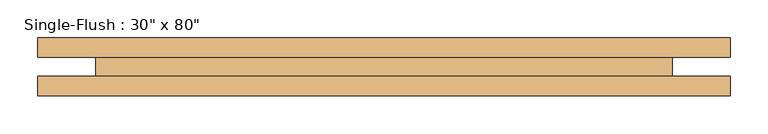
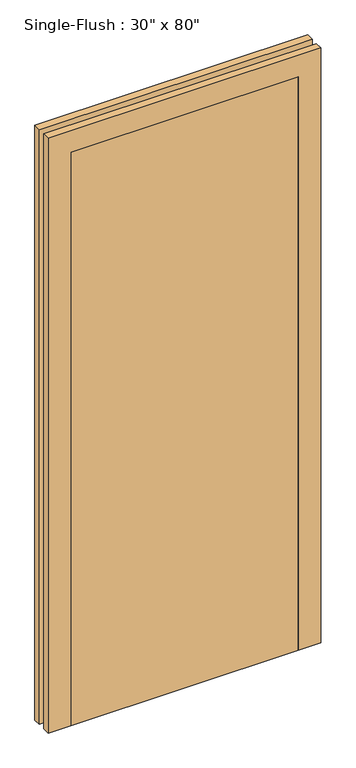
"""IFC4 building model written with IfcOpenShell, lengths in millimetres: door geometry."""

from ifc_helpers import new_model, si_unit, frame, origin, origin_with_axes, place, context, project, spatial, polyline, outline, extrude, source, transform, mapped, element, save


def door_b03708da(model_context):
    return source(origin(), model_context, "Body", "SweptSolid", [
        extrude(outline(polyline([(2108.2, -457.2), (0.0, -457.2), (0.0, -381.0), (2032.0, -381.0), (2032.0, 381.0), (0.0, 381.0), (0.0, 457.2), (2108.2, 457.2), (2108.2, -457.2)])), frame((0.0, 12.7, 0.0), z_axis=(0.0, 1.0, 0.0), x_axis=(0.0, 0.0, 1.0)), (0.0, 0.0, 1.0), 25.4),
        extrude(outline(polyline([(2108.2, 457.2), (2108.2, -457.2), (0.0, -457.2), (0.0, -381.0), (2032.0, -381.0), (2032.0, 381.0), (0.0, 381.0), (0.0, 457.2), (2108.2, 457.2)])), frame((0.0, -38.1, 0.0), z_axis=(0.0, 1.0, 0.0), x_axis=(0.0, 0.0, 1.0)), (0.0, 0.0, 1.0), 25.4),
        extrude(outline(polyline([(381.0, -38.1), (-381.0, -38.1), (-381.0, 12.7), (381.0, 12.7), (381.0, -38.1)])), origin_with_axes(), (0.0, 0.0, 1.0), 2032.0),
    ])


if __name__ == "__main__":
    model = new_model("IFC4")
    model_context = context("Model", 3, world=origin())
    ifc_project = project(units=[si_unit("LENGTHUNIT", "METRE", prefix="MILLI")], contexts=[model_context])
    site = spatial("IfcSite", under=ifc_project)
    building = spatial("IfcBuilding", under=site)
    placement = place(None, origin())
    door_shape = door_b03708da(model_context)
    element("IfcDoor", 1, ObjectType="Single-Flush : 30\" x 80\"", at=placement, inside=building, context=model_context, shape_type="MappedRepresentation", body=[
        mapped(door_shape, transform((0.0, 0.0, 0.0), x_axis=(1.0, 0.0, 0.0), y_axis=(0.0, 1.0, 0.0), z_axis=(0.0, 0.0, 1.0))),
    ])
    save(model, "model.ifc")

# Revit data of these elements
# Type "Single-Flush : 30\" x 80\""
#   Type Mark = "5"
#   Construction Type Id = "MDOOR"
#   Assembly Code = "C1020"
#   Analytic Construction = "Metal"
#   Thickness = 0' - 2"
#   Heat Transfer Coefficient (U) = 0.651978 BTU/(h·ft²·°F)
#   Height = 6' - 8"
#   Trim Projection Ext = 0' - 1"
#   Trim Projection Int = 0' - 1"
#   Trim Width = 0' - 3"
#   Width = 2' - 6"
#   Define Thermal Properties by = 1
#   Define Thermal Properties by = 1
#   Door Material = Door - Panel
#   Frame Material = Door - Frame
#   Visual Light Transmittance = 0
#   Solar Heat Gain Coefficient = 0
#   Function = (empty or 0)
#   Wall Closure = (empty or 0)
# Element 1 (IfcDoor, "Single-Flush : 30\" x 80\"")
#   Materials on its faces: "Door - Frame", "Door - Panel"
# Materials
#   "Door - Panel": class "Wood", colour RGB 210 159 95, transparency 0, Cost = 0
#   "Door - Frame": class "Miscellaneous", colour RGB 118 70 51, transparency 0, Cost = 0
